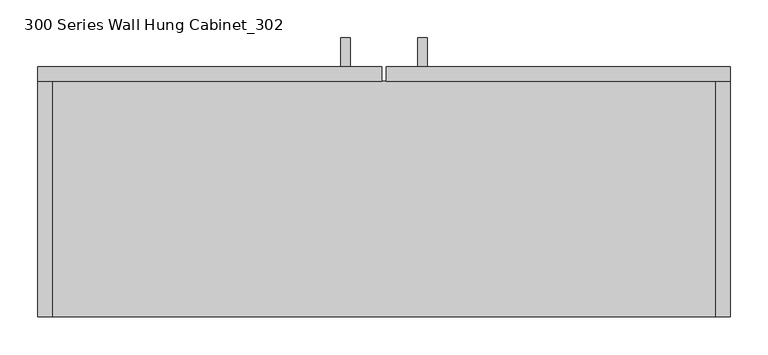
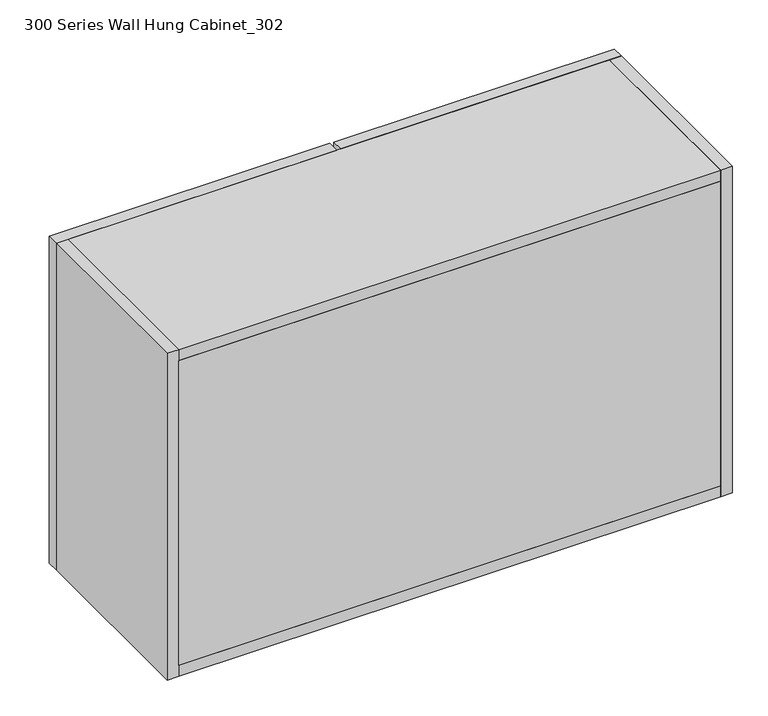
"""IFC4 building model written with IfcOpenShell, lengths in millimetres: furniture geometry, 300 Series Wall Hung Cabinet_302."""

from ifc_helpers import new_model, si_unit, frame, origin, place, context, project, spatial, polyline, outline, extrude, source, transform, mapped, element, save


def furniture_300_series_wall_hung_cabinet_302_73f347b2(model_context):
    return source(origin(), model_context, "Body", "SweptSolid", [
        extrude(outline(polyline([(406.4, 1708.1425373), (406.4, 1720.8121874), (444.4810937, 1720.8121874), (444.4810937, 1625.6), (406.4, 1625.6), (406.4, 1638.2696501), (431.8114436, 1638.2696501), (431.8114436, 1708.1425373), (406.4, 1708.1425373)])), frame((-57.15, 0.0, 0.0), z_axis=(1.0, 0.0, 0.0), x_axis=(0.0, 1.0, 0.0)), (0.0, 0.0, 1.0), 12.4065288),
        extrude(outline(polyline([(406.4, 1708.1425373), (406.4, 1720.8121874), (444.4810937, 1720.8121874), (444.4810937, 1625.6), (406.4, 1625.6), (406.4, 1638.2696501), (431.8114436, 1638.2696501), (431.8114436, 1708.1425373), (406.4, 1708.1425373)])), frame((44.45, 0.0, 0.0), z_axis=(1.0, 0.0, 0.0), x_axis=(0.0, 1.0, 0.0)), (0.0, 0.0, 1.0), 12.4065288),
        extrude(outline(polyline([(438.15, 76.2), (-438.15, 76.2), (-438.15, 95.25), (438.15, 95.25), (438.15, 76.2)])), frame((0.0, 0.0, 1593.85), z_axis=(0.0, 0.0, 1.0), x_axis=(1.0, 0.0, 0.0)), (0.0, 0.0, 1.0), 520.7),
        extrude(outline(polyline([(-3.175, 387.35), (-457.2, 387.35), (-457.2, 406.4), (-3.175, 406.4), (-3.175, 387.35)])), frame((0.0, 0.0, 1574.8), z_axis=(0.0, 0.0, 1.0), x_axis=(1.0, 0.0, 0.0)), (0.0, 0.0, 1.0), 558.8),
        extrude(outline(polyline([(457.2, 387.35), (3.175, 387.35), (3.175, 406.4), (457.2, 406.4), (457.2, 387.35)])), frame((0.0, 0.0, 1574.8), z_axis=(0.0, 0.0, 1.0), x_axis=(1.0, 0.0, 0.0)), (0.0, 0.0, 1.0), 558.8),
        extrude(outline(polyline([(-457.2, 76.2), (-457.2, 387.35), (-438.15, 387.35), (-438.15, 76.2), (-457.2, 76.2)])), frame((0.0, 0.0, 1574.8), z_axis=(0.0, 0.0, 1.0), x_axis=(1.0, 0.0, 0.0)), (0.0, 0.0, 1.0), 558.8),
        extrude(outline(polyline([(438.15, 76.2), (438.15, 387.35), (457.2, 387.35), (457.2, 76.2), (438.15, 76.2)])), frame((0.0, 0.0, 1574.8), z_axis=(0.0, 0.0, 1.0), x_axis=(1.0, 0.0, 0.0)), (0.0, 0.0, 1.0), 558.8),
        extrude(outline(polyline([(438.15, 387.35), (438.15, 76.2), (-438.15, 76.2), (-438.15, 387.35), (438.15, 387.35)])), frame((0.0, 0.0, 2114.55), z_axis=(0.0, 0.0, 1.0), x_axis=(1.0, 0.0, 0.0)), (0.0, 0.0, 1.0), 19.05),
        extrude(outline(polyline([(438.15, 387.35), (438.15, 76.2), (-438.15, 76.2), (-438.15, 387.35), (438.15, 387.35)])), frame((0.0, 0.0, 1574.8), z_axis=(0.0, 0.0, 1.0), x_axis=(1.0, 0.0, 0.0)), (0.0, 0.0, 1.0), 19.05),
    ])


if __name__ == "__main__":
    model = new_model("IFC4")
    model_context = context("Model", 3, world=origin())
    ifc_project = project(units=[si_unit("LENGTHUNIT", "METRE", prefix="MILLI")], contexts=[model_context])
    site = spatial("IfcSite", under=ifc_project)
    building = spatial("IfcBuilding", under=site)
    placement = place(None, origin())
    furniture_300_series_wall_hung_cabinet_302_shape = furniture_300_series_wall_hung_cabinet_302_73f347b2(model_context)
    element("IfcFurniture", 1, ObjectType="300 Series Wall Hung Cabinet_302 : 36\"W x 21\"H", at=placement, inside=building, context=model_context, shape_type="MappedRepresentation", body=[
        mapped(furniture_300_series_wall_hung_cabinet_302_shape, transform((0.0, 0.0, 0.0), x_axis=(1.0, 0.0, 0.0), y_axis=(0.0, 1.0, 0.0), z_axis=(0.0, 0.0, 1.0))),
    ])
    save(model, "model.ifc")

# Revit data of these elements
# Type "300 Series Wall Hung Cabinet_302 : 36\"W x 21\"H"
#   URL = "www.wicnet.org/manual_sections.asp"
#   Model = "302"
#   Manufacturer = "Woodwork Institute"
#   Description = "Wall Hung Cabinet"
#   Content Creator URL = "www.AECcontent.com"
#   Content Creator = "AECcontent"
#   Assembly Code = "E2010200"
#   Width = 3' - 0"
#   Top of Cabinet = 7' - 0"
#   Height = 1' - 10"
#   Depth = 1' - 1"
#   Top Panel Material = Cabinet
#   Side Panel Material = Cabinet
#   Shelf Panel Material = Cabinet
#   Door Panel Material = Cabinet
# Element 1 (IfcFurniture, "300 Series Wall Hung Cabinet_302 : 36\"W x 21\"H")
#   Materials on its faces: "Cabinet", "Default metal"
# Materials
#   "Cabinet": class "Wood", colour RGB 189 170 130, transparency 0, Cost = 0
#   "Default metal": class "Unassigned", colour RGB 204 204 204, transparency 0
